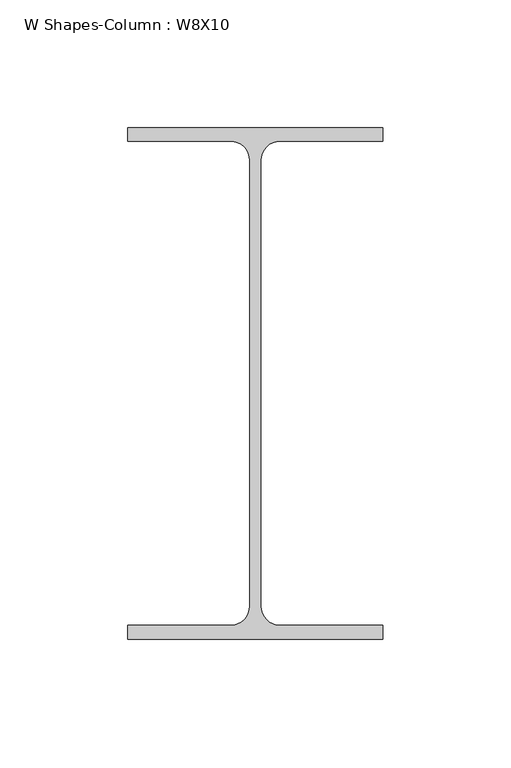
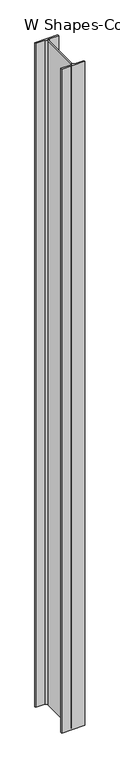
"""IFC4 building model written with IfcOpenShell, lengths in millimetres: column geometry, W Shapes-Column : W8X10."""

from ifc_helpers import new_model, si_unit, point, frame_2d, origin, origin_with_axes, place, context, project, spatial, polyline, circle_curve, trimmed, segment, composite_curve, outline, extrude, source, transform, mapped, element, save


def w_shapes_column_w8x10_fd6cb265(model_context):
    return source(origin(), model_context, "Body", "SweptSolid", [
        extrude(outline(composite_curve([segment(polyline([(50.038, 100.203), (50.038, 94.869), (9.779, 94.869)]), True, "CONTINUOUS"), segment(trimmed(circle_curve(frame_2d((9.779, 87.249)), 7.62), [point((9.779, 94.869))], [point((2.159, 87.249))], True, "CARTESIAN"), True, "CONTINUOUS"), segment(polyline([(2.159, 87.249), (2.159, -87.249)]), True, "CONTINUOUS"), segment(trimmed(circle_curve(frame_2d((9.779, -87.249)), 7.62), [point((2.159, -87.249))], [point((9.779, -94.869))], True, "CARTESIAN"), True, "CONTINUOUS"), segment(polyline([(9.779, -94.869), (50.038, -94.869), (50.038, -100.203), (-50.038, -100.203), (-50.038, -94.869), (-9.779, -94.869)]), True, "CONTINUOUS"), segment(trimmed(circle_curve(frame_2d((-9.779, -87.249)), 7.62), [point((-9.779, -94.869))], [point((-2.159, -87.249))], True, "CARTESIAN"), True, "CONTINUOUS"), segment(polyline([(-2.159, -87.249), (-2.159, 87.249)]), True, "CONTINUOUS"), segment(trimmed(circle_curve(frame_2d((-9.779, 87.249)), 7.62), [point((-2.159, 87.249))], [point((-9.779, 94.869))], True, "CARTESIAN"), True, "CONTINUOUS"), segment(polyline([(-9.779, 94.869), (-50.038, 94.869), (-50.038, 100.203), (50.038, 100.203)]), True, "CONTINUOUS")], self_intersect=False)), origin_with_axes(), (0.0, 0.0, 1.0), 3048.0),
    ])


if __name__ == "__main__":
    model = new_model("IFC4")
    model_context = context("Model", 3, world=origin())
    ifc_project = project(units=[si_unit("LENGTHUNIT", "METRE", prefix="MILLI")], contexts=[model_context])
    site = spatial("IfcSite", under=ifc_project)
    building = spatial("IfcBuilding", under=site)
    placement = place(None, origin())
    w_shapes_column_w8x10_shape = w_shapes_column_w8x10_fd6cb265(model_context)
    element("IfcColumn", 1, ObjectType="W Shapes-Column : W8X10", at=placement, inside=building, context=model_context, shape_type="MappedRepresentation", body=[
        mapped(w_shapes_column_w8x10_shape, transform((0.0, 0.0, 0.0), x_axis=(1.0, 0.0, 0.0), y_axis=(0.0, 1.0, 0.0), z_axis=(0.0, 0.0, 1.0))),
    ])
    save(model, "model.ifc")

# Revit data of these elements
# Type "W Shapes-Column : W8X10"
#   Section Name Key = "W8x10"
#   Assembly Code = "B10"
#   Width = 100.076 mm
#   Web Thickness = 4.318 mm
#   Web Fillet = 7.62 mm
#   Warping Constant = 8297.76 cm⁶
#   Torsional Moment of Inertia = 1.77315 cm⁴
#   Section Area = 2.96 in²
#   Plastic Modulus weak axis = 0.000960648 (stored number, unit not read)
#   Plastic Modulus strong axis = 0.0051331 (stored number, unit not read)
#   Perimeter = 9.35736 m²/m
#   Nominal Weight = 145.939 N/m
#   Moment of Inertia weak axis = 86.9924 cm⁴
#   Moment of Inertia strong axis = 1281.99 cm⁴
#   Height = 200.406 mm
#   Flange Thickness = 5.334 mm
#   Elastic Modulus weak axis = 0.000613426 (stored number, unit not read)
#   Elastic Modulus strong axis = 0.00451968 (stored number, unit not read)
#   Centroid Vertical = 100.203 mm
#   Centroid Horizontal = 50.038 mm
#   Structural Material [instance default] = Steel ASTM A992
#   Principal Axes Angle = 0
# Element 1 (IfcColumn, "W Shapes-Column : W8X10")
#   Materials on its faces: "Steel ASTM A992"
# Materials
#   "Steel ASTM A992": class "Metal", colour RGB 199 199 199, transparency 0, Description = "Structural steel 50ksi", Cost = 0
